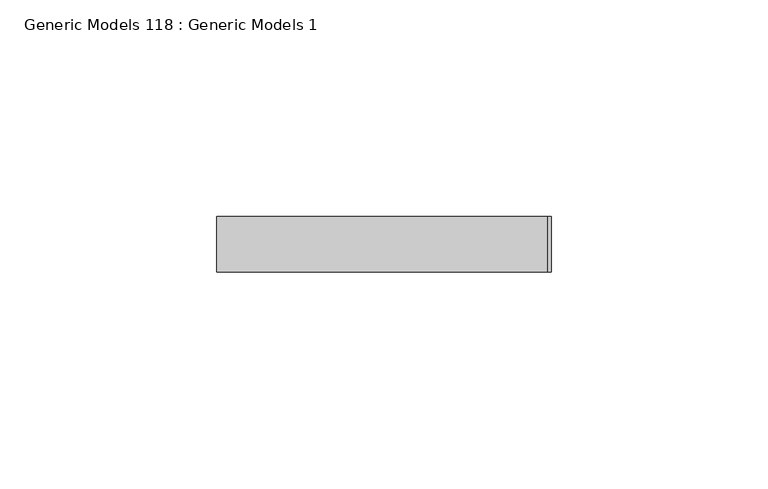
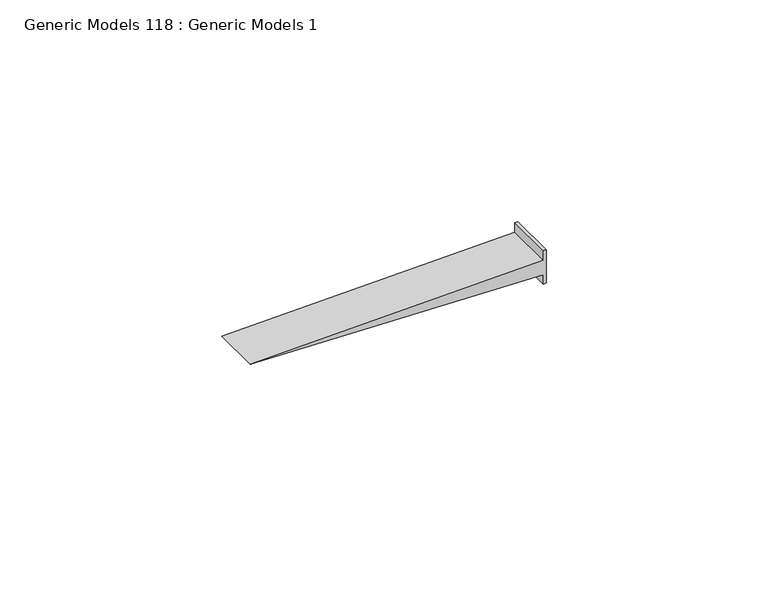
"""IFC4 building model written with IfcOpenShell, lengths in millimetres: proxy geometry, Generic Models 118 : Generic Models 1."""

from ifc_helpers import new_model, si_unit, frame, origin, place, context, project, spatial, polyline, outline, extrude, source, transform, mapped, element, save


def generic_models_118_generic_models_1_9632d76d(model_context):
    return source(origin(), model_context, "Body", "SweptSolid", [
        extrude(outline(polyline([(2414.3721662, 49800.66875), (2414.3721662, 49799.875), (2411.8223026, 49799.875), (2409.8255662, 49723.675), (2407.8288298, 49799.875), (2405.2789662, 49799.875), (2405.2789662, 49800.66875), (2414.3721662, 49800.66875)])), frame((0.0, 565.15, 0.0), z_axis=(0.0, 1.0, 0.0), x_axis=(0.0, 0.0, 1.0)), (0.0, 0.0, 1.0), 12.7),
    ])


if __name__ == "__main__":
    model = new_model("IFC4")
    model_context = context("Model", 3, world=origin())
    ifc_project = project(units=[si_unit("LENGTHUNIT", "METRE", prefix="MILLI")], contexts=[model_context])
    site = spatial("IfcSite", under=ifc_project)
    building = spatial("IfcBuilding", under=site)
    placement = place(None, origin())
    generic_models_118_generic_models_1_shape = generic_models_118_generic_models_1_9632d76d(model_context)
    element("IfcBuildingElementProxy", 1, Name="Generic Models 118 : Generic Models 1", ObjectType="Generic Models 118 : Generic Models 1", at=placement, inside=building, context=model_context, shape_type="MappedRepresentation", body=[
        mapped(generic_models_118_generic_models_1_shape, transform((0.0, 0.0, 0.0), x_axis=(1.0, 0.0, 0.0), y_axis=(0.0, 1.0, 0.0), z_axis=(0.0, 0.0, 1.0))),
    ])
    save(model, "model.ifc")

# Revit data of these elements
# Element 1 (IfcBuildingElementProxy, "Generic Models 118 : Generic Models 1")
#   Materials on its faces: "ATTACH GYPSUM BOARD TO STUDS AND NOT TO TOP TRACK"
# Materials
#   "ATTACH GYPSUM BOARD TO STUDS AND NOT TO TOP TRACK": class "Generic", colour RGB 48 48 48, transparency 0, Cost = 0
